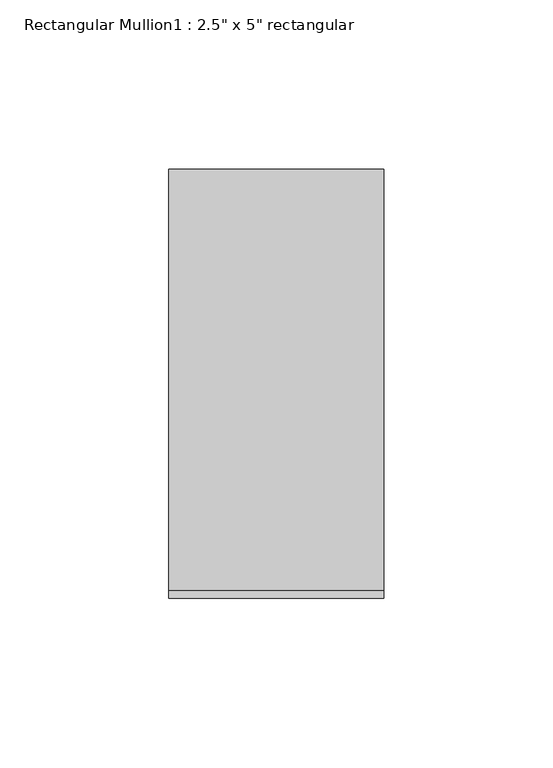
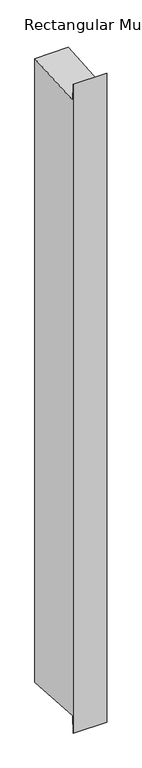
"""IFC4 building model written with IfcOpenShell, lengths in millimetres: member geometry."""

from ifc_helpers import new_model, si_unit, frame, origin, place, context, project, spatial, polyline, outline, extrude, source, transform, mapped, element, save


def member_60f38ea1(model_context):
    return source(origin(), model_context, "Body", "SweptSolid", [
        extrude(outline(polyline([(-63.5, 29.6036678), (-61.2111885, -4.2153013), (63.5, 4.2249441), (63.5, -1253.4859011), (-61.2111885, -1245.0456557), (-63.5, -1278.8646248), (-63.5, 29.6036678)])), frame((-63.5, 0.0, 0.0), z_axis=(1.0, 0.0, 0.0), x_axis=(0.0, 1.0, 0.0)), (0.0, 0.0, 1.0), 63.5),
    ])


if __name__ == "__main__":
    model = new_model("IFC4")
    model_context = context("Model", 3, world=origin())
    ifc_project = project(units=[si_unit("LENGTHUNIT", "METRE", prefix="MILLI")], contexts=[model_context])
    site = spatial("IfcSite", under=ifc_project)
    building = spatial("IfcBuilding", under=site)
    placement = place(None, origin())
    member_shape = member_60f38ea1(model_context)
    element("IfcMember", 1, ObjectType="Rectangular Mullion1 : 2.5\" x 5\" rectangular", at=placement, inside=building, context=model_context, shape_type="MappedRepresentation", body=[
        mapped(member_shape, transform((0.0, 0.0, 0.0), x_axis=(1.0, 0.0, 0.0), y_axis=(0.0, 1.0, 0.0), z_axis=(0.0, 0.0, 1.0))),
    ])
    save(model, "model.ifc")

# Revit data of these elements
# Type "Rectangular Mullion1 : 2.5\" x 5\" rectangular"
#   built-in parameter 1007304 = 0.416667 (stored number, unit not read)
#   built-in parameter 1007301 = 0.104167 (stored number, unit not read)
#   built-in parameter 1007300 = 0.104167 (stored number, unit not read)
# Element 1 (IfcMember, "Rectangular Mullion1 : 2.5\" x 5\" rectangular")
#   Materials on its faces: "support-frame"
# Materials
#   "support-frame": class "Unassigned", colour RGB 233 233 233, transparency 0, Cost = 0
